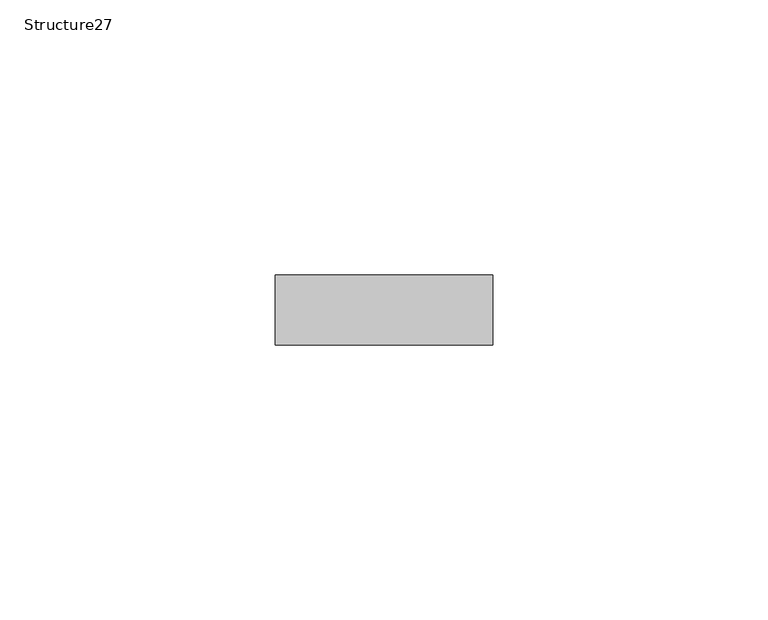
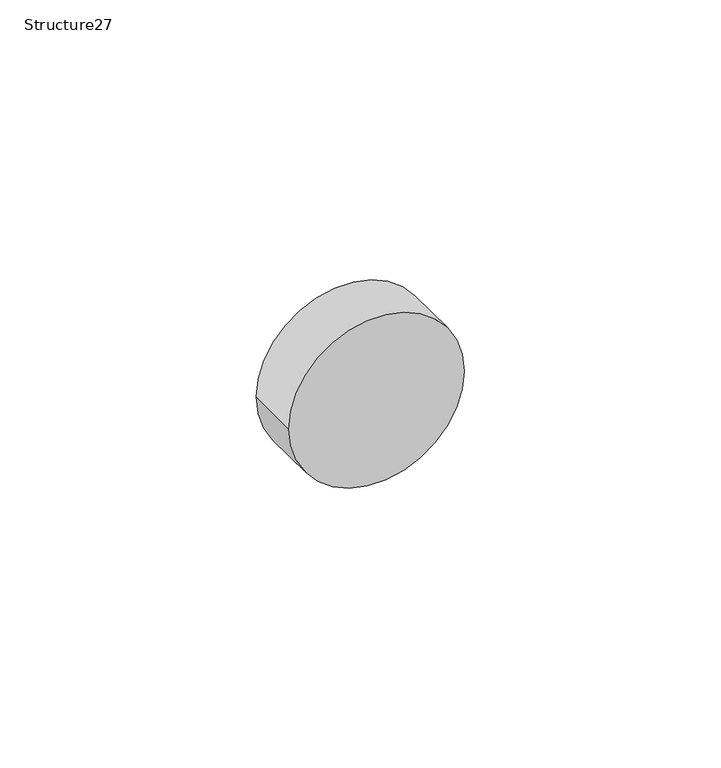
"""IFC4 building model written with IfcOpenShell, lengths in millimetres: proxy geometry, Structure27 : Structure668217125."""

from ifc_helpers import new_model, si_unit, point, frame, frame_2d, origin, place, context, project, spatial, circle_curve, trimmed, segment, composite_curve, outline, extrude, source, transform, mapped, element, save


def structure27_ed8abd19(model_context):
    return source(origin(), model_context, "Body", "SweptSolid", [
        extrude(outline(composite_curve([segment(trimmed(circle_curve(frame_2d((39371.6422813, 7343.0332877)), 19.7708678), [point((39371.6422813, 7323.2624199))], [point((39371.6422813, 7362.8041555))], False, "CARTESIAN"), True, "CONTINUOUS"), segment(trimmed(circle_curve(frame_2d((39371.6422813, 7343.0332877)), 19.7708678), [point((39371.6422813, 7362.8041555))], [point((39371.6422813, 7323.2624199))], False, "CARTESIAN"), True, "CONTINUOUS")], self_intersect=False)), frame((0.0, 920.8121669, 0.0), z_axis=(0.0, 1.0, 0.0), x_axis=(0.0, 0.0, 1.0)), (0.0, 0.0, 1.0), 12.7),
    ])


if __name__ == "__main__":
    model = new_model("IFC4")
    model_context = context("Model", 3, world=origin())
    ifc_project = project(units=[si_unit("LENGTHUNIT", "METRE", prefix="MILLI")], contexts=[model_context])
    site = spatial("IfcSite", under=ifc_project)
    building = spatial("IfcBuilding", under=site)
    placement = place(None, origin())
    structure27_shape = structure27_ed8abd19(model_context)
    element("IfcBuildingElementProxy", 1, Name="Structure27 : Structure668217125", ObjectType="Structure27 : Structure668217125", at=placement, inside=building, context=model_context, shape_type="MappedRepresentation", body=[
        mapped(structure27_shape, transform((0.0, 0.0, 0.0), x_axis=(1.0, 0.0, 0.0), y_axis=(0.0, 1.0, 0.0), z_axis=(0.0, 0.0, 1.0))),
    ])
    save(model, "model.ifc")

# Revit data of these elements
# Type "Structure27 : Structure668217125"
#   NameOverride = "Structure668217125"
# Element 1 (IfcBuildingElementProxy, "Structure27 : Structure668217125")
#   Materials on its faces: "1.5\" DIA. STAINLESS STEEL RAILING"
# Materials
#   "1.5\" DIA. STAINLESS STEEL RAILING": class "Unassigned", colour RGB 128 128 128, transparency 0, Cost = 0
